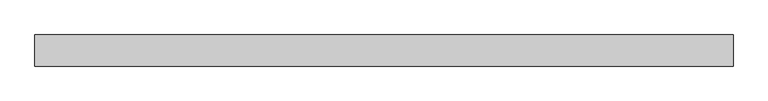
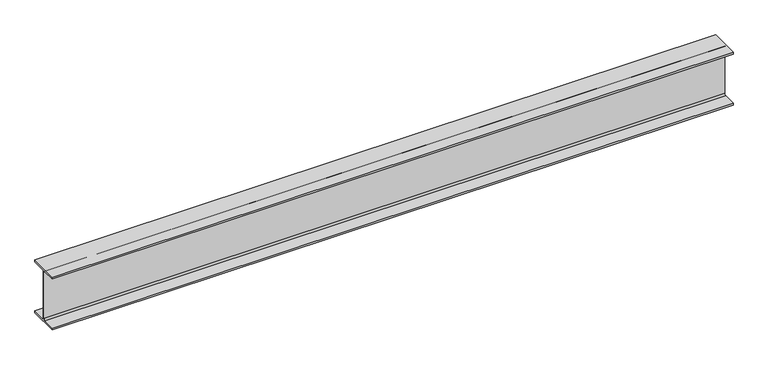
"""IFC4 building model written with IfcOpenShell, lengths in millimetres: beam geometry, Old_Steel Beam_H-KSD3502 : H_SB_ASB_H-200×200x8x12."""

from ifc_helpers import new_model, si_unit, point, frame, frame_2d, origin, place, context, project, spatial, polyline, circle_curve, trimmed, segment, composite_curve, outline, extrude, source, transform, mapped, element, save


def beam_0d3d728d(model_context):
    return source(origin(), model_context, "Body", "SweptSolid", [
        extrude(outline(composite_curve([segment(polyline([(82.5, -141.5), (82.5, -151.7), (-82.5, -151.7), (-82.5, -141.5), (-11.9, -141.5)]), True, "CONTINUOUS"), segment(trimmed(circle_curve(frame_2d((-11.9, -132.6)), 8.9), [point((-11.9, -141.5))], [point((-3.0, -132.6))], True, "CARTESIAN"), True, "CONTINUOUS"), segment(polyline([(-3.0, -132.6), (-3.0, 132.6)]), True, "CONTINUOUS"), segment(trimmed(circle_curve(frame_2d((-11.9, 132.6)), 8.9), [point((-3.0, 132.6))], [point((-11.9, 141.5))], True, "CARTESIAN"), True, "CONTINUOUS"), segment(polyline([(-11.9, 141.5), (-82.5, 141.5), (-82.5, 151.7), (82.5, 151.7), (82.5, 141.5), (11.9, 141.5)]), True, "CONTINUOUS"), segment(trimmed(circle_curve(frame_2d((11.9, 132.6)), 8.9), [point((11.9, 141.5))], [point((3.0, 132.6))], True, "CARTESIAN"), True, "CONTINUOUS"), segment(polyline([(3.0, 132.6), (3.0, -132.6)]), True, "CONTINUOUS"), segment(trimmed(circle_curve(frame_2d((11.9, -132.6)), 8.9), [point((3.0, -132.6))], [point((11.9, -141.5))], True, "CARTESIAN"), True, "CONTINUOUS"), segment(polyline([(11.9, -141.5), (82.5, -141.5)]), True, "CONTINUOUS")], self_intersect=False)), frame((-1887.2000261, 0.0, 0.0), z_axis=(1.0, 0.0, 0.0), x_axis=(0.0, 1.0, 0.0)), (0.0, 0.0, 1.0), 3702.1907618),
    ])


if __name__ == "__main__":
    model = new_model("IFC4")
    model_context = context("Model", 3, world=origin())
    ifc_project = project(units=[si_unit("LENGTHUNIT", "METRE", prefix="MILLI")], contexts=[model_context])
    site = spatial("IfcSite", under=ifc_project)
    building = spatial("IfcBuilding", under=site)
    placement = place(None, origin())
    beam_shape = beam_0d3d728d(model_context)
    element("IfcBeam", 1, ObjectType="Old_Steel Beam_H-KSD3502 : H_SB_ASB_H-200×200x8x12", at=placement, inside=building, context=model_context, shape_type="MappedRepresentation", body=[
        mapped(beam_shape, transform((0.0, 0.0, 0.0), x_axis=(1.0, 0.0, 0.0), y_axis=(0.0, 1.0, 0.0), z_axis=(0.0, 0.0, 1.0))),
    ])
    save(model, "model.ifc")

# Revit data of these elements
# Type "Old_Steel Beam_H-KSD3502 : H_SB_ASB_H-200×200x8x12"
#   Width = 20.0 cm
#   Web Thickness = 0.8 cm
#   Web Fillet = 1.3 cm
#   Warping Constant = 141376.0 cm⁶
#   Torsional Moment of Inertia = 26.2485 cm⁴
#   Torsional Modulus = 1.0 cm³
#   Section Area = 63.53 cm²
#   Plastic Modulus weak axis = 244.0 cm³
#   Plastic Modulus strong axis = 525.0 cm³
#   Perimeter = 1.16 m²/m
#   Nominal Weight = 49.90 kgf/m
#   Moment of Inertia weak axis = 1600.00 cm⁴
#   Moment of Inertia strong axis = 4720.00 cm⁴
#   Height = 20.0 cm
#   Flange Thickness = 1.2 cm
#   Elastic Modulus weak axis = 160.0 cm³
#   Elastic Modulus strong axis = 472.0 cm³
#   Centroid Vertical = 10.0 cm
#   Centroid Horizontal = 10.0 cm
#   Length [instance default] = 1.5240 m
#   Structural Material [instance default] = Steel, 45-345
#   Assembly Code = ""
# Element 1 (IfcBeam, "Old_Steel Beam_H-KSD3502 : H_SB_ASB_H-200×200x8x12")
#   Structural Material = none
# Materials
#   "Steel, 45-345": class "Metal", colour RGB 189 187 185, transparency 0, Description = "Steel 345 MPa", Cost = 0
